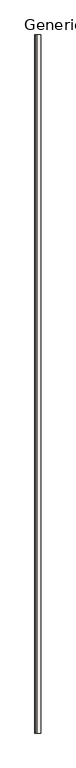
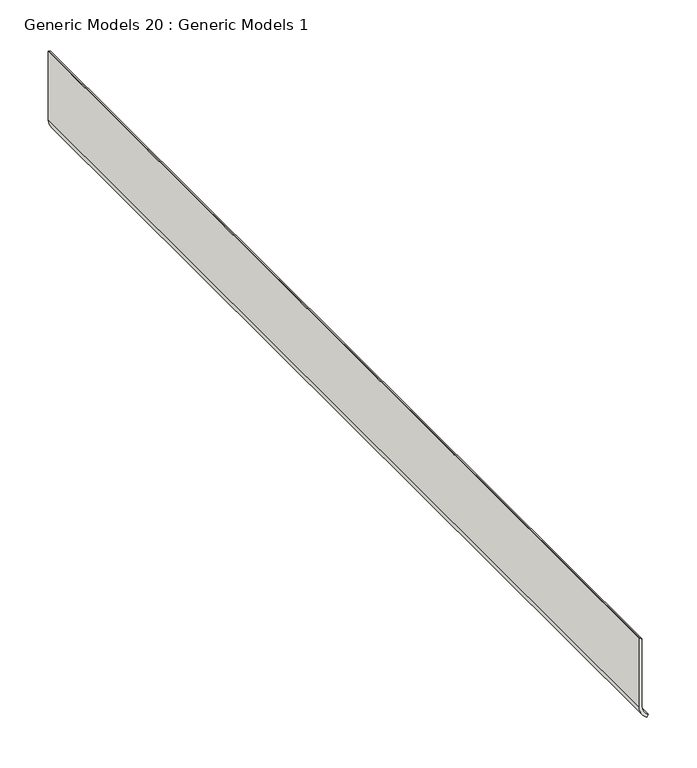
"""IFC4 building model written with IfcOpenShell, lengths in millimetres: wall geometry, Generic Models 20 : Generic Models 1."""

from ifc_helpers import new_model, si_unit, point, frame, frame_2d, origin, place, context, project, spatial, polyline, circle_curve, trimmed, segment, composite_curve, outline, extrude, source, transform, mapped, element, save


def generic_models_20_generic_models_1_ef70466a(model_context):
    return source(origin(), model_context, "Body", "SweptSolid", [
        extrude(outline(composite_curve([segment(polyline([(101.6, 49799.875), (15.4496307, 49799.875)]), True, "CONTINUOUS"), segment(trimmed(circle_curve(frame_2d((15.4496307, 49817.7146968)), 17.8396968), [point((15.4496307, 49799.875))], [point((0.0, 49808.7948484))], False, "CARTESIAN"), True, "CONTINUOUS"), segment(polyline([(0.0, 49808.7948484), (2.7496307, 49810.3823484)]), True, "CONTINUOUS"), segment(trimmed(circle_curve(frame_2d((15.4496307, 49817.7146968)), 14.6646968), [point((2.7496307, 49810.3823484))], [point((15.4496307, 49803.05))], True, "CARTESIAN"), True, "CONTINUOUS"), segment(polyline([(15.4496307, 49803.05), (99.5131982, 49803.05)]), True, "CONTINUOUS"), segment(trimmed(circle_curve(frame_2d((99.5131982, 49800.9631982)), 2.0868018), [point((99.5131982, 49803.05))], [point((101.6, 49800.9631982))], False, "CARTESIAN"), True, "CONTINUOUS"), segment(polyline([(101.6, 49800.9631982), (101.6, 49799.875)]), True, "CONTINUOUS")], self_intersect=False)), frame((0.0, 0.0, 0.0), z_axis=(0.0, 1.0, 0.0), x_axis=(0.0, 0.0, 1.0)), (0.0, 0.0, 1.0), 1219.2),
    ])


if __name__ == "__main__":
    model = new_model("IFC4")
    model_context = context("Model", 3, world=origin())
    ifc_project = project(units=[si_unit("LENGTHUNIT", "METRE", prefix="MILLI")], contexts=[model_context])
    site = spatial("IfcSite", under=ifc_project)
    building = spatial("IfcBuilding", under=site)
    placement = place(None, origin())
    generic_models_20_generic_models_1_shape = generic_models_20_generic_models_1_ef70466a(model_context)
    element("IfcWall", 1, ObjectType="Generic Models 20 : Generic Models 1", at=placement, inside=building, context=model_context, shape_type="MappedRepresentation", body=[
        mapped(generic_models_20_generic_models_1_shape, transform((0.0, 0.0, 0.0), x_axis=(1.0, 0.0, 0.0), y_axis=(0.0, 1.0, 0.0), z_axis=(0.0, 0.0, 1.0))),
    ])
    save(model, "model.ifc")

# Revit data of these elements
# Element 1 (IfcWall, "Generic Models 20 : Generic Models 1")
#   Materials on its faces: "WALL BASE AS SCHEDULED"
# Materials
#   "WALL BASE AS SCHEDULED": class "Generic", colour RGB 120 120 120, transparency 0, Cost = 0
